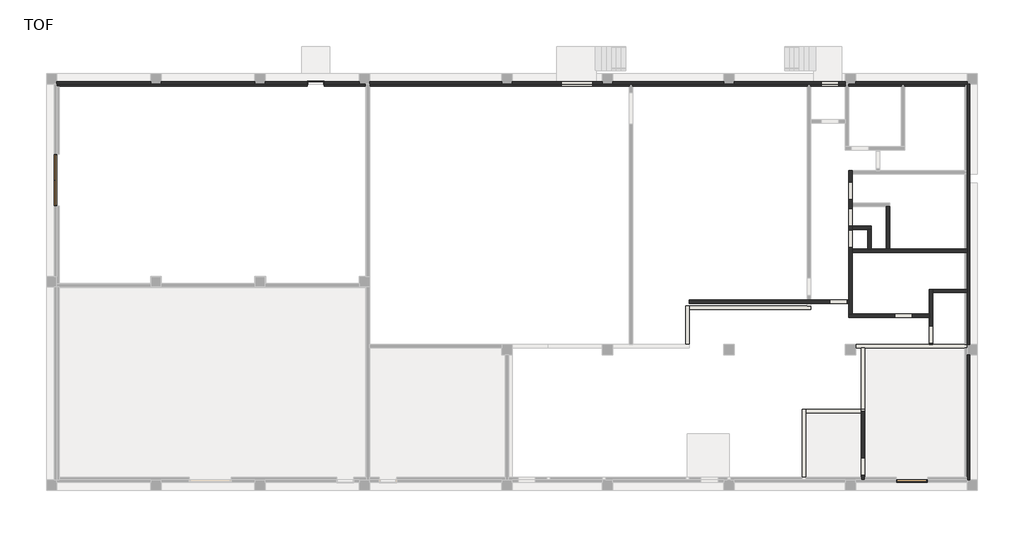
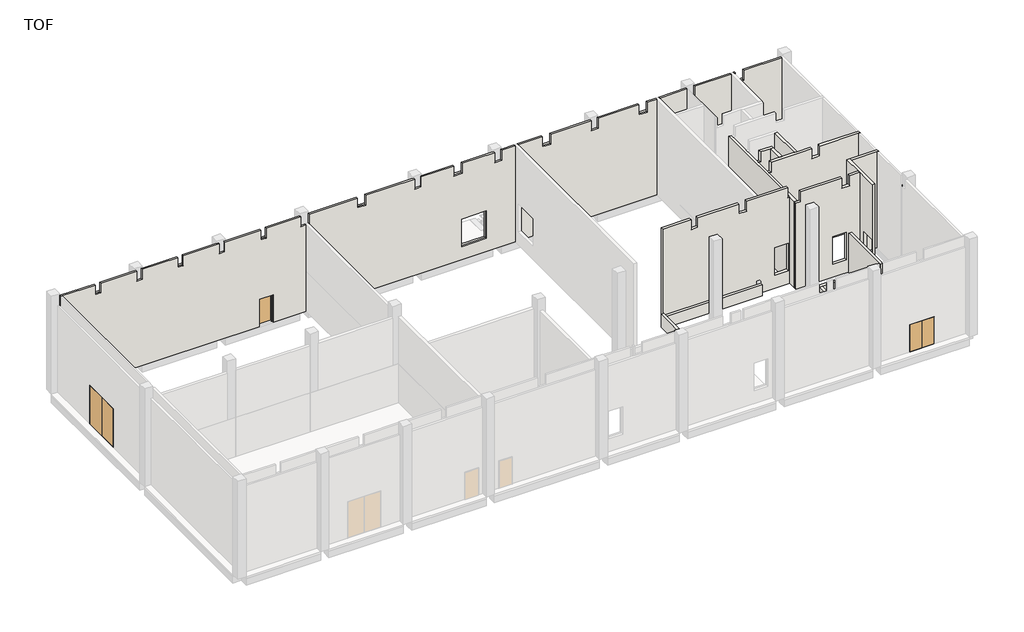
# One storey, part 2 of 4: 19 walls, 3 doors.
"""IFC4 building model written with IfcOpenShell, lengths in millimetres."""

import ifcopenshell
import ifcopenshell.guid

model = None  # the IFC model being written
_history = None  # IfcOwnerHistory: only IFC2X3 demands one
_inside = {}  # id of a spatial element -> (the spatial element, [elements in it])
_under = {}  # id of a project, library or spatial element -> (it, [spatial elements below it])
_declared = {}  # id of a project -> (the project, [libraries it declares])
_typed = {}  # id of a type object -> (the type object, [elements of that type])
_made_of = {}  # id of a material, layer set ... -> (it, [elements and type objects made of it])


def new_model(schema):
    """Start an empty IFC model of exactly this schema.

    Asked for "IFC4X3", IfcOpenShell would pick the latest addendum, in which some entities
    have other attributes; the version numbers below select the first issue.
    IFC2X3 requires an IfcOwnerHistory on every rooted entity: one is made here for all.
    """
    global model, _history
    if schema == "IFC4X3":
        model = ifcopenshell.file(schema_version=(4, 3, 0, 0))
    else:
        model = ifcopenshell.file(schema=schema)
    _inside.clear()
    _under.clear()
    _declared.clear()
    _typed.clear()
    _made_of.clear()
    _history = None
    if model.schema == "IFC2X3":
        org = make("IfcOrganization", Name="unknown")
        user = make(
            "IfcPersonAndOrganization",
            ThePerson=make("IfcPerson", FamilyName="unknown"),
            TheOrganization=org,
        )
        app = make(
            "IfcApplication",
            ApplicationDeveloper=org,
            Version="unknown",
            ApplicationFullName="unknown",
            ApplicationIdentifier="unknown",
        )
        _history = make(
            "IfcOwnerHistory",
            OwningUser=user,
            OwningApplication=app,
            ChangeAction="ADDED",
            CreationDate=0,
        )
    return model


def make(cls, **values):
    """One entity of the class cls with the attributes given. An attribute that is None is left unset."""
    return model.create_entity(
        cls, **{name: value for name, value in values.items() if value is not None}
    )


def rooted(cls, **values):
    """An entity with a GlobalId (a new one), such as an element, a storey or a relation."""
    return make(cls, GlobalId=ifcopenshell.guid.new(), OwnerHistory=_history, **values)


def si_unit(unit_type, name, prefix=None):
    """IfcSIUnit, for example si_unit("LENGTHUNIT", "METRE", prefix="MILLI")."""
    return make("IfcSIUnit", UnitType=unit_type, Prefix=prefix, Name=name)


def assignment(units):
    """IfcUnitAssignment: the units of a project."""
    return None if units is None else make("IfcUnitAssignment", Units=units)


def point(xyz):
    """IfcCartesianPoint."""
    return None if xyz is None else make("IfcCartesianPoint", Coordinates=xyz)


def direction(xyz):
    """IfcDirection."""
    return None if xyz is None else make("IfcDirection", DirectionRatios=xyz)


def frame(location, z_axis=None, x_axis=None):
    """IfcAxis2Placement3D, a coordinate frame: its origin and axes. An axis left out is left unset."""
    return make(
        "IfcAxis2Placement3D",
        Location=point(location),
        Axis=direction(z_axis),
        RefDirection=direction(x_axis),
    )


def origin():
    """The frame at (0, 0, 0) with its axes left unset."""
    return frame((0.0, 0.0, 0.0))


def origin_with_axes():
    """The frame at (0, 0, 0) with the z axis (0, 0, 1) and the x axis (1, 0, 0) written out."""
    return frame((0.0, 0.0, 0.0), z_axis=(0.0, 0.0, 1.0), x_axis=(1.0, 0.0, 0.0))


def place(relative_to, where):
    """IfcLocalPlacement: puts the frame where relative to a parent placement (None: the world)."""
    return make(
        "IfcLocalPlacement", PlacementRelTo=relative_to, RelativePlacement=where
    )


def context(
    kind, dimensions, precision=None, world=None, true_north=None, identifier=None
):
    """IfcGeometricRepresentationContext, for example the 3D "Model" context."""
    return make(
        "IfcGeometricRepresentationContext",
        ContextIdentifier=identifier,
        ContextType=kind,
        CoordinateSpaceDimension=dimensions,
        Precision=precision,
        WorldCoordinateSystem=world,
        TrueNorth=true_north,
    )


def project(units=None, contexts=None):
    """IfcProject with its units and contexts."""
    return rooted(
        "IfcProject",
        Name="project",
        RepresentationContexts=contexts,
        UnitsInContext=assignment(units),
    )


def spatial(cls, under=None, at=None, **own):
    """A site, building, storey or space (cls), placed at a placement, below another one or the project."""
    s = rooted(cls, ObjectPlacement=at, **own)
    if under is not None:
        _under.setdefault(under.id(), (under, []))[1].append(s)
    return s


def polyline(points):
    """IfcPolyline through the points."""
    return make("IfcPolyline", Points=[point(p) for p in points])


def outline(outer, holes=None, kind="AREA"):
    """IfcArbitraryClosedProfileDef: a profile drawn as a closed curve; with holes, ...WithVoids."""
    if holes is None:
        return make("IfcArbitraryClosedProfileDef", ProfileType=kind, OuterCurve=outer)
    return make(
        "IfcArbitraryProfileDefWithVoids",
        ProfileType=kind,
        OuterCurve=outer,
        InnerCurves=holes,
    )


def extrude(swept, where, along, depth):
    """IfcExtrudedAreaSolid: the profile swept, set in the frame where, extruded along a direction by depth."""
    return make(
        "IfcExtrudedAreaSolid",
        SweptArea=swept,
        Position=where,
        ExtrudedDirection=direction(along),
        Depth=depth,
    )


def faces_of(points, faces, orient=None, outer=None):
    """IfcFace entities. A face is a list of loops; a loop is a list of indices into points, from 0.

    orient and outer hold one flag for each loop. By default every Orientation is true, the
    first loop of a face is its IfcFaceOuterBound and the others are IfcFaceBound.
    """
    made = []
    for i, loops in enumerate(faces):
        bounds = []
        for j, loop in enumerate(loops):
            is_outer = j == 0 if outer is None else outer[i][j]
            bounds.append(
                make(
                    "IfcFaceOuterBound" if is_outer else "IfcFaceBound",
                    Bound=make("IfcPolyLoop", Polygon=[points[k] for k in loop]),
                    Orientation=True if orient is None else orient[i][j],
                )
            )
        made.append(make("IfcFace", Bounds=bounds))
    return made


def faceted_brep(points, faces, orient=None, outer=None, voids=None):
    """IfcFacetedBrep: a solid bounded by flat faces; with voids (closed shells), ...WithVoids."""
    shared = [point(p) for p in points]
    hull = make("IfcClosedShell", CfsFaces=faces_of(shared, faces, orient, outer))
    if voids is None:
        return make("IfcFacetedBrep", Outer=hull)
    return make(
        "IfcFacetedBrepWithVoids",
        Outer=hull,
        Voids=[
            make(cls, CfsFaces=faces_of(shared, fs, o, b)) for cls, fs, o, b in voids
        ],
    )


def shape(context_of_items, identifier, shape_type, items):
    """IfcShapeRepresentation: the items that make up one representation, for example the "Body"."""
    return make(
        "IfcShapeRepresentation",
        ContextOfItems=context_of_items,
        RepresentationIdentifier=identifier,
        RepresentationType=shape_type,
        Items=items,
    )


def source(mapping_origin, context_of_items, identifier, shape_type, items):
    """IfcRepresentationMap: a shape defined once, which mapped items show again and again."""
    return make(
        "IfcRepresentationMap",
        MappingOrigin=mapping_origin,
        MappedRepresentation=shape(context_of_items, identifier, shape_type, items),
    )


def transform(
    local_origin,
    x_axis=None,
    y_axis=None,
    z_axis=None,
    scale=None,
    scale2=None,
    scale3=None,
    uniform=True,
):
    """IfcCartesianTransformationOperator3D, or its non-uniform kind. x_axis, y_axis, z_axis: its Axis1, 2, 3."""
    if uniform:
        return make(
            "IfcCartesianTransformationOperator3D",
            Axis1=direction(x_axis),
            Axis2=direction(y_axis),
            LocalOrigin=point(local_origin),
            Scale=scale,
            Axis3=direction(z_axis),
        )
    return make(
        "IfcCartesianTransformationOperator3DnonUniform",
        Axis1=direction(x_axis),
        Axis2=direction(y_axis),
        LocalOrigin=point(local_origin),
        Scale=scale,
        Axis3=direction(z_axis),
        Scale2=scale2,
        Scale3=scale3,
    )


def mapped(mapping_source, mapping_target):
    """IfcMappedItem: shows the shape of a source again, moved by a transform."""
    return make(
        "IfcMappedItem", MappingSource=mapping_source, MappingTarget=mapping_target
    )


def made_of(thing, what):
    """Note that an element or type object is made of a material, layer set ...; save() writes the relation."""
    if what is not None:
        _made_of.setdefault(what.id(), (what, []))[1].append(thing)
    return thing


def element(
    cls,
    number,
    at=None,
    inside=None,
    cuts=None,
    type_object=None,
    material=None,
    context=None,
    identifier="Body",
    shape_type=None,
    held_by="IfcProductDefinitionShape",
    body=None,
    shapes=None,
    **own,
):
    """One element of the class cls, such as IfcWall. Its Tag is "e" and its number.

    at: its placement. inside: the storey or other place that contains it. cuts: it is an
    opening in that element (IfcRelVoidsElement). A single representation is given by context,
    identifier, shape_type and body (its items); several are given by shapes. held_by: the class
    of the entity that holds the representations. save() writes the other relations.
    """
    e = rooted(cls, Tag="e%d" % number, ObjectPlacement=at, **own)
    if body is not None:
        shapes = [shape(context, identifier, shape_type, body)]
    if shapes is not None:
        e.Representation = make(held_by, Representations=shapes)
    if inside is not None:
        _inside.setdefault(inside.id(), (inside, []))[1].append(e)
    if cuts is not None:
        rooted(
            "IfcRelVoidsElement", RelatingBuildingElement=cuts, RelatedOpeningElement=e
        )
    if type_object is not None:
        _typed.setdefault(type_object.id(), (type_object, []))[1].append(e)
    return made_of(e, material)


def aggregate(whole, parts):
    """IfcRelAggregates: a whole, such as a stair, and the parts it consists of."""
    return rooted("IfcRelAggregates", RelatingObject=whole, RelatedObjects=parts)


def save(model, path):
    """Write the relations noted so far, then the file.

    IfcRelAggregates (storeys below a building ...), IfcRelContainedInSpatialStructure (elements
    in a storey), IfcRelDefinesByType, IfcRelAssociatesMaterial and IfcRelDeclares: one each for
    every whole, place, type object, material and project.
    """
    for whole, parts in _under.values():
        aggregate(whole, parts)
    for where, things in _inside.values():
        rooted(
            "IfcRelContainedInSpatialStructure",
            RelatedElements=things,
            RelatingStructure=where,
        )
    for kind, things in _typed.values():
        rooted("IfcRelDefinesByType", RelatedObjects=things, RelatingType=kind)
    for what, things in _made_of.values():
        rooted("IfcRelAssociatesMaterial", RelatedObjects=things, RelatingMaterial=what)
    for by, libraries in _declared.values():
        rooted("IfcRelDeclares", RelatingContext=by, RelatedDefinitions=libraries)
    model.write(path)


def double_door_steel_580823b0(model_context):
    return source(origin(), model_context, "Body", "SolidModel", [
        extrude(outline(polyline([(880.0, 35.0), (0.0, 35.0), (0.0, 75.0), (880.0, 75.0), (880.0, 35.0)])), frame((0.0, 0.0, 20.0), z_axis=(0.0, 0.0, 1.0), x_axis=(1.0, 0.0, 0.0)), (0.0, 0.0, 1.0), 2060.0),
        extrude(outline(polyline([(0.0, 35.0), (-880.0, 35.0), (-880.0, 75.0), (0.0, 75.0), (0.0, 35.0)])), frame((0.0, 0.0, 20.0), z_axis=(0.0, 0.0, 1.0), x_axis=(1.0, 0.0, 0.0)), (0.0, 0.0, 1.0), 2060.0),
        faceted_brep([(900.0, -75.0, 2100.0), (900.0, 75.0, 2100.0), (-900.0, 75.0, 2100.0), (-900.0, -75.0, 2100.0), (865.0, 35.0, 2065.0), (865.0, -75.0, 2065.0), (-865.0, -75.0, 2065.0), (-865.0, 35.0, 2065.0), (880.0, 75.0, 2080.0), (880.0, 35.0, 2080.0), (-880.0, 35.0, 2080.0), (-880.0, 75.0, 2080.0), (-900.0, 75.0, 0.0), (-900.0, -75.0, 0.0), (-865.0, -75.0, 35.0), (-865.0, 35.0, 35.0), (-880.0, 35.0, 20.0), (-880.0, 75.0, 20.0), (900.0, 75.0, 0.0), (880.0, 75.0, 20.0), (900.0, -75.0, 0.0), (865.0, -75.0, 35.0), (865.0, 35.0, 35.0), (880.0, 35.0, 20.0)], [[[0, 1, 2, 3]], [[4, 5, 6, 7]], [[8, 9, 10, 11]], [[3, 2, 12, 13]], [[7, 6, 14, 15]], [[11, 10, 16, 17]], [[18, 12, 2, 1], [8, 11, 17, 19]], [[13, 12, 18, 20]], [[0, 3, 13, 20], [21, 14, 6, 5]], [[15, 14, 21, 22]], [[23, 16, 10, 9], [4, 7, 15, 22]], [[17, 16, 23, 19]], [[20, 18, 1, 0]], [[22, 21, 5, 4]], [[19, 23, 9, 8]]]),
    ])


def double_door_steel_0432cfbf(model_context):
    return source(origin(), model_context, "Body", "SolidModel", [
        extrude(outline(polyline([(1480.0, 35.0), (0.0, 35.0), (0.0, 75.0), (1480.0, 75.0), (1480.0, 35.0)])), frame((0.0, 0.0, 20.0), z_axis=(0.0, 0.0, 1.0), x_axis=(1.0, 0.0, 0.0)), (0.0, 0.0, 1.0), 2960.0),
        extrude(outline(polyline([(0.0, 35.0), (-1480.0, 35.0), (-1480.0, 75.0), (0.0, 75.0), (0.0, 35.0)])), frame((0.0, 0.0, 20.0), z_axis=(0.0, 0.0, 1.0), x_axis=(1.0, 0.0, 0.0)), (0.0, 0.0, 1.0), 2960.0),
        faceted_brep([(1500.0, -75.0, 3000.0), (1500.0, 75.0, 3000.0), (-1500.0, 75.0, 3000.0), (-1500.0, -75.0, 3000.0), (1465.0, 35.0, 2965.0), (1465.0, -75.0, 2965.0), (-1465.0, -75.0, 2965.0), (-1465.0, 35.0, 2965.0), (1480.0, 75.0, 2980.0), (1480.0, 35.0, 2980.0), (-1480.0, 35.0, 2980.0), (-1480.0, 75.0, 2980.0), (-1500.0, 75.0, 0.0), (-1500.0, -75.0, 0.0), (-1465.0, -75.0, 35.0), (-1465.0, 35.0, 35.0), (-1480.0, 35.0, 20.0), (-1480.0, 75.0, 20.0), (1500.0, 75.0, 0.0), (1480.0, 75.0, 20.0), (1500.0, -75.0, 0.0), (1465.0, -75.0, 35.0), (1465.0, 35.0, 35.0), (1480.0, 35.0, 20.0)], [[[0, 1, 2, 3]], [[4, 5, 6, 7]], [[8, 9, 10, 11]], [[3, 2, 12, 13]], [[7, 6, 14, 15]], [[11, 10, 16, 17]], [[18, 12, 2, 1], [8, 11, 17, 19]], [[13, 12, 18, 20]], [[0, 3, 13, 20], [21, 14, 6, 5]], [[15, 14, 21, 22]], [[23, 16, 10, 9], [4, 7, 15, 22]], [[17, 16, 23, 19]], [[20, 18, 1, 0]], [[22, 21, 5, 4]], [[19, 23, 9, 8]]]),
    ])


def single_door_steel_8d57826b(model_context):
    return source(origin(), model_context, "Body", "SolidModel", [
        extrude(outline(polyline([(470.0, -105.0), (-470.0, -105.0), (-470.0, -70.0), (470.0, -70.0), (470.0, -105.0)])), origin_with_axes(), (0.0, 0.0, 1.0), 2070.0),
        faceted_brep([(470.0, -105.0, 0.0), (470.0, -70.0, 0.0), (450.0, -70.0, 0.0), (450.0, 70.0, 0.0), (470.0, 70.0, 0.0), (470.0, 105.0, 0.0), (500.0, 105.0, 0.0), (500.0, -105.0, 0.0), (500.0, -105.0, 2100.0), (-500.0, -105.0, 2100.0), (-500.0, -105.0, 0.0), (-470.0, -105.0, 0.0), (-470.0, -105.0, 2070.0), (470.0, -105.0, 2070.0), (500.0, 105.0, 2100.0), (470.0, 105.0, 2070.0), (-470.0, 105.0, 2070.0), (-470.0, 105.0, 0.0), (-500.0, 105.0, 0.0), (-500.0, 105.0, 2100.0), (470.0, 70.0, 2070.0), (450.0, 70.0, 2050.0), (-450.0, 70.0, 2050.0), (-450.0, 70.0, 0.0), (-470.0, 70.0, 0.0), (-470.0, 70.0, 2070.0), (450.0, -70.0, 2050.0), (470.0, -70.0, 2070.0), (-470.0, -70.0, 2070.0), (-470.0, -70.0, 0.0), (-450.0, -70.0, 0.0), (-450.0, -70.0, 2050.0)], [[[0, 1, 2, 3, 4, 5, 6, 7]], [[7, 8, 9, 10, 11, 12, 13, 0]], [[6, 14, 8, 7]], [[5, 15, 16, 17, 18, 19, 14, 6]], [[4, 20, 15, 5]], [[3, 21, 22, 23, 24, 25, 20, 4]], [[2, 26, 21, 3]], [[1, 27, 28, 29, 30, 31, 26, 2]], [[0, 13, 27, 1]], [[12, 11, 29, 28]], [[11, 10, 18, 17, 24, 23, 30, 29]], [[19, 18, 10, 9]], [[25, 24, 17, 16]], [[31, 30, 23, 22]], [[14, 19, 9, 8]], [[20, 25, 16, 15]], [[26, 31, 22, 21]], [[13, 12, 28, 27]]]),
    ])


model = new_model("IFC4")

# Units and contexts
model_context = context("Model", 3, world=origin())
ifc_project = project(units=[si_unit("LENGTHUNIT", "METRE", prefix="MILLI")], contexts=[model_context])

# Site, building, storey
site = spatial("IfcSite", under=ifc_project)
building = spatial("IfcBuilding", under=site)
storey = spatial("IfcBuildingStorey", under=building, Name="TOF", Elevation=149.9618634)

# Doors
placement = place(None, origin())
double_door_steel_shape = double_door_steel_580823b0(model_context)
element("IfcDoor", 1, ObjectType="Double Door_Steel : H_DR_AR_B12_Double Door_Steel_W2000xH2100", at=placement, inside=storey, context=model_context, shape_type="MappedRepresentation", body=[
    mapped(double_door_steel_shape, transform((49525.0, 724.5208589, 149.9618634), x_axis=(-1.0, 0.0, 0.0), y_axis=(0.0, -1.0, 0.0), z_axis=(0.0, 0.0, 1.0))),
])
double_door_steel_2_shape = double_door_steel_0432cfbf(model_context)
element("IfcDoor", 2, ObjectType="Double Door_Steel : H_DR_AR_B12_Double Door_Steel_W3000xH3000", at=placement, inside=storey, context=model_context, shape_type="MappedRepresentation", body=[
    mapped(double_door_steel_2_shape, transform((225.0, 18074.5208589, 149.9618634), x_axis=(0.0, 1.0, 0.0), y_axis=(-1.0, 0.0, 0.0), z_axis=(0.0, 0.0, 1.0))),
])
single_door_steel_shape = single_door_steel_8d57826b(model_context)
element("IfcDoor", 3, ObjectType="Single Door_Steel : H_DR_AR_B12_Single Door_Steel_W1000xH2100", at=placement, inside=storey, context=model_context, shape_type="MappedRepresentation", body=[
    mapped(single_door_steel_shape, transform((15200.0, 23674.5208589, 149.9618634), x_axis=(-1.0, 0.0, 0.0), y_axis=(0.0, -1.0, 0.0), z_axis=(0.0, 0.0, 1.0))),
])

# Walls
element("IfcWall", 4, ObjectType="H_WA_AR_B02_Ext Wall_RC T150", at=placement, inside=storey, context=model_context, shape_type="Brep", body=[
    faceted_brep([(14700.0, 23599.5208589, 149.9618634), (14700.0, 23599.5208589, 2249.9618634), (15700.0, 23599.5208589, 2249.9618634), (15700.0, 23599.5208589, 149.9618634), (17700.0, 23599.5208589, 149.9618634), (17700.0, 23599.5208589, 6749.9618634), (15200.0, 23599.5208589, 6749.9618634), (14800.0, 23599.5208589, 6749.9618634), (12300.0, 23599.5208589, 6749.9618634), (12300.0, 23599.5208589, 149.9618634), (14700.0, 23749.5208589, 2249.9618634), (14700.0, 23749.5208589, 149.9618634), (12300.0, 23749.5208589, 149.9618634), (12300.0, 23749.5208589, 6749.9618634), (17700.0, 23749.5208589, 6749.9618634), (17700.0, 23749.5208589, 149.9618634), (15700.0, 23749.5208589, 149.9618634), (15700.0, 23749.5208589, 2249.9618634)], [[[0, 1, 2, 3, 4, 5, 6, 7, 8, 9]], [[10, 11, 12, 13, 14, 15, 16, 17]], [[11, 0, 9, 12]], [[3, 16, 15, 4]], [[10, 1, 0, 11]], [[1, 10, 17, 2]], [[2, 17, 16, 3]], [[12, 9, 8, 13]], [[4, 15, 14, 5]], [[8, 7, 6, 5, 14, 13]]]),
    faceted_brep([(300.0, 23599.5208589, 149.9618634), (5700.0, 23599.5208589, 149.9618634), (5700.0, 23599.5208589, 6749.9618634), (3200.0, 23599.5208589, 6749.9618634), (2800.0, 23599.5208589, 6749.9618634), (300.0, 23599.5208589, 6749.9618634), (5700.0, 23749.5208589, 149.9618634), (300.0, 23749.5208589, 149.9618634), (300.0, 23749.5208589, 6749.9618634), (5700.0, 23749.5208589, 6749.9618634)], [[[0, 1, 2, 3, 4, 5]], [[6, 7, 8, 9]], [[0, 7, 6, 1]], [[7, 0, 5, 8]], [[1, 6, 9, 2]], [[5, 4, 3, 2, 9, 8]]]),
    faceted_brep([(6300.0, 23599.5208589, 149.9618634), (11700.0, 23599.5208589, 149.9618634), (11700.0, 23599.5208589, 6749.9618634), (9200.0, 23599.5208589, 6749.9618634), (8800.0, 23599.5208589, 6749.9618634), (6300.0, 23599.5208589, 6749.9618634), (11700.0, 23749.5208589, 149.9618634), (6300.0, 23749.5208589, 149.9618634), (6300.0, 23749.5208589, 6749.9618634), (11700.0, 23749.5208589, 6749.9618634)], [[[0, 1, 2, 3, 4, 5]], [[6, 7, 8, 9]], [[0, 7, 6, 1]], [[7, 0, 5, 8]], [[1, 6, 9, 2]], [[5, 4, 3, 2, 9, 8]]]),
    faceted_brep([(18300.0, 23599.5208589, 149.9618634), (25900.0, 23599.5208589, 149.9618634), (25900.0, 23599.5208589, 6749.9618634), (22400.0, 23599.5208589, 6749.9618634), (21800.0, 23599.5208589, 6749.9618634), (18300.0, 23599.5208589, 6749.9618634), (25900.0, 23749.5208589, 149.9618634), (18300.0, 23749.5208589, 149.9618634), (18300.0, 23749.5208589, 6749.9618634), (25900.0, 23749.5208589, 6749.9618634)], [[[0, 1, 2, 3, 4, 5]], [[6, 7, 8, 9]], [[0, 7, 6, 1]], [[7, 0, 5, 8]], [[1, 6, 9, 2]], [[5, 4, 3, 2, 9, 8]]]),
    faceted_brep([(26500.0, 23599.5208589, 149.9618634), (31700.0, 23599.5208589, 149.9618634), (31700.0, 23599.5208589, 6749.9618634), (29400.0, 23599.5208589, 6749.9618634), (28800.0, 23599.5208589, 6749.9618634), (26500.0, 23599.5208589, 6749.9618634), (31150.0, 23599.5208589, 3249.9618634), (31150.0, 23599.5208589, 1149.9618634), (29350.0, 23599.5208589, 1149.9618634), (29350.0, 23599.5208589, 3249.9618634), (31700.0, 23749.5208589, 149.9618634), (26500.0, 23749.5208589, 149.9618634), (26500.0, 23749.5208589, 6749.9618634), (31700.0, 23749.5208589, 6749.9618634), (31150.0, 23749.5208589, 1149.9618634), (31150.0, 23749.5208589, 3249.9618634), (29350.0, 23749.5208589, 3249.9618634), (29350.0, 23749.5208589, 1149.9618634)], [[[0, 1, 2, 3, 4, 5], [6, 7, 8, 9]], [[10, 11, 12, 13], [14, 15, 16, 17]], [[0, 11, 10, 1]], [[15, 14, 7, 6]], [[16, 15, 6, 9]], [[17, 16, 9, 8]], [[14, 17, 8, 7]], [[11, 0, 5, 12]], [[1, 10, 13, 2]], [[5, 4, 3, 2, 13, 12]]]),
    faceted_brep([(32300.0, 23599.5208589, 149.9618634), (33250.0, 23599.5208589, 149.9618634), (33450.0, 23599.5208589, 149.9618634), (38700.0, 23599.5208589, 149.9618634), (38700.0, 23599.5208589, 6749.9618634), (35800.0, 23599.5208589, 6749.9618634), (35200.0, 23599.5208589, 6749.9618634), (32300.0, 23599.5208589, 6749.9618634), (38700.0, 23749.5208589, 149.9618634), (32300.0, 23749.5208589, 149.9618634), (32300.0, 23749.5208589, 6749.9618634), (38700.0, 23749.5208589, 6749.9618634)], [[[0, 1, 2, 3, 4, 5, 6, 7]], [[8, 9, 10, 11]], [[0, 9, 8, 3, 2, 1]], [[9, 0, 7, 10]], [[3, 8, 11, 4]], [[7, 6, 5, 4, 11, 10]]]),
    faceted_brep([(39300.0, 23599.5208589, 149.9618634), (43500.0, 23599.5208589, 149.9618634), (43700.0, 23599.5208589, 149.9618634), (45700.0, 23599.5208589, 149.9618634), (45700.0, 23599.5208589, 6749.9618634), (42800.0, 23599.5208589, 6749.9618634), (42200.0, 23599.5208589, 6749.9618634), (39300.0, 23599.5208589, 6749.9618634), (44300.0, 23599.5208589, 1149.9618634), (44300.0, 23599.5208589, 3249.9618634), (45300.0, 23599.5208589, 3249.9618634), (45300.0, 23599.5208589, 1149.9618634), (45700.0, 23749.5208589, 149.9618634), (39300.0, 23749.5208589, 149.9618634), (39300.0, 23749.5208589, 6749.9618634), (45700.0, 23749.5208589, 6749.9618634), (44300.0, 23749.5208589, 3249.9618634), (44300.0, 23749.5208589, 1149.9618634), (45300.0, 23749.5208589, 1149.9618634), (45300.0, 23749.5208589, 3249.9618634)], [[[0, 1, 2, 3, 4, 5, 6, 7], [8, 9, 10, 11]], [[12, 13, 14, 15], [16, 17, 18, 19]], [[0, 13, 12, 3, 2, 1]], [[9, 8, 17, 16]], [[10, 9, 16, 19]], [[11, 10, 19, 18]], [[8, 11, 18, 17]], [[13, 0, 7, 14]], [[3, 12, 15, 4]], [[7, 6, 5, 4, 15, 14]]]),
    faceted_brep([(46300.0, 23599.5208589, 149.9618634), (48900.0, 23599.5208589, 149.9618634), (49100.0, 23599.5208589, 149.9618634), (52574.0, 23599.5208589, 149.9618634), (52700.0, 23599.5208589, 149.9618634), (52700.0, 23599.5208589, 6749.9618634), (49800.0, 23599.5208589, 6749.9618634), (49200.0, 23599.5208589, 6749.9618634), (46300.0, 23599.5208589, 6749.9618634), (52700.0, 23749.5208589, 149.9618634), (46300.0, 23749.5208589, 149.9618634), (46300.0, 23749.5208589, 6749.9618634), (52700.0, 23749.5208589, 6749.9618634)], [[[0, 1, 2, 3, 4, 5, 6, 7, 8]], [[9, 10, 11, 12]], [[9, 4, 3, 2, 1, 0, 10]], [[4, 9, 12, 5]], [[10, 0, 8, 11]], [[8, 7, 6, 5, 12, 11]]]),
])
element("IfcWall", 5, ObjectType="H_WA_AR_B02_Ext Wall_RC T150", at=placement, inside=storey, context=model_context, shape_type="Brep", body=[
    faceted_brep([(52700.0, 7999.5208589, 149.9618634), (52700.0, 925.5208589, 149.9618634), (52700.0, 799.5208589, 149.9618634), (52700.0, 799.5208589, 6749.9618634), (52700.0, 7999.5208589, 6749.9618634), (52850.0, 799.5208589, 149.9618634), (52850.0, 7999.5208589, 149.9618634), (52850.0, 7999.5208589, 6749.9618634), (52850.0, 799.5208589, 6749.9618634)], [[[0, 1, 2, 3, 4]], [[5, 6, 7, 8]], [[5, 2, 1, 0, 6]], [[2, 5, 8, 3]], [[6, 0, 4, 7]], [[4, 3, 8, 7]]]),
    faceted_brep([(52700.0, 23599.5208589, 149.9618634), (52700.0, 18599.5208589, 149.9618634), (52700.0, 18399.5208589, 149.9618634), (52700.0, 17899.5208589, 149.9618634), (52700.0, 14099.5208589, 149.9618634), (52700.0, 13899.5208589, 149.9618634), (52700.0, 11774.5208589, 149.9618634), (52700.0, 11574.5208589, 149.9618634), (52700.0, 8599.5208589, 149.9618634), (52700.0, 8599.5208589, 6749.9618634), (52700.0, 23599.5208589, 6749.9618634), (52850.0, 8599.5208589, 149.9618634), (52850.0, 23599.5208589, 149.9618634), (52850.0, 23599.5208589, 6749.9618634), (52850.0, 8599.5208589, 6749.9618634)], [[[0, 1, 2, 3, 4, 5, 6, 7, 8, 9, 10]], [[11, 12, 13, 14]], [[0, 12, 11, 8, 7, 6, 5, 4, 3, 2, 1]], [[12, 0, 10, 13]], [[8, 11, 14, 9]], [[10, 9, 14, 13]]]),
])
element("IfcWall", 6, ObjectType="H_WA_AR_B02_Int Wall_Block T200", at=placement, inside=storey, context=model_context, shape_type="Brep", body=[
    faceted_brep([(36700.0, 10949.5208589, 149.9618634), (45895.0, 10949.5208589, 149.9618634), (45895.0, 10949.5208589, 6749.9618634), (45750.0, 10949.5208589, 6749.9618634), (45750.0, 10949.5208589, 7499.9618634), (42800.0, 10949.5208589, 7499.9618634), (42800.0, 10949.5208589, 6749.9618634), (42200.0, 10949.5208589, 6749.9618634), (42200.0, 10949.5208589, 7499.9618634), (39250.0, 10949.5208589, 7499.9618634), (39250.0, 10949.5208589, 6749.9618634), (38750.0, 10949.5208589, 6749.9618634), (38750.0, 10949.5208589, 7499.9618634), (36700.0, 10949.5208589, 7499.9618634), (44800.0, 10949.5208589, 1149.9618634), (44800.0, 10949.5208589, 3249.9618634), (45800.0, 10949.5208589, 3249.9618634), (45800.0, 10949.5208589, 1149.9618634), (45895.0, 11149.5208589, 149.9618634), (43700.0, 11149.5208589, 149.9618634), (43500.0, 11149.5208589, 149.9618634), (36700.0, 11149.5208589, 149.9618634), (36700.0, 11149.5208589, 1149.9618634), (36700.0, 11149.5208589, 7499.9618634), (38750.0, 11149.5208589, 7499.9618634), (38750.0, 11149.5208589, 6749.9618634), (39250.0, 11149.5208589, 6749.9618634), (39250.0, 11149.5208589, 7499.9618634), (42200.0, 11149.5208589, 7499.9618634), (42200.0, 11149.5208589, 6749.9618634), (42800.0, 11149.5208589, 6749.9618634), (42800.0, 11149.5208589, 7499.9618634), (43500.0, 11149.5208589, 7499.9618634), (43700.0, 11149.5208589, 7499.9618634), (45750.0, 11149.5208589, 7499.9618634), (45750.0, 11149.5208589, 6749.9618634), (45895.0, 11149.5208589, 6749.9618634), (44800.0, 11149.5208589, 3249.9618634), (44800.0, 11149.5208589, 1149.9618634), (45800.0, 11149.5208589, 1149.9618634), (45800.0, 11149.5208589, 3249.9618634)], [[[0, 1, 2, 3, 4, 5, 6, 7, 8, 9, 10, 11, 12, 13], [14, 15, 16, 17]], [[18, 19, 20, 21, 22, 23, 24, 25, 26, 27, 28, 29, 30, 31, 32, 33, 34, 35, 36], [37, 38, 39, 40]], [[1, 0, 21, 20, 19, 18]], [[21, 0, 13, 23, 22]], [[1, 18, 36, 2]], [[15, 14, 38, 37]], [[16, 15, 37, 40]], [[17, 16, 40, 39]], [[14, 17, 39, 38]], [[26, 10, 9, 27]], [[10, 26, 25, 11]], [[11, 25, 24, 12]], [[35, 3, 2, 36]], [[3, 35, 34, 4]], [[7, 29, 28, 8]], [[29, 7, 6, 30]], [[30, 6, 5, 31]], [[5, 4, 34, 33, 32, 31]], [[9, 8, 28, 27]], [[13, 12, 24, 23]]]),
])
element("IfcWall", 7, ObjectType="H_WA_AR_B02_Int Wall_Block T200", at=placement, inside=storey, context=model_context, shape_type="Brep", body=[
    faceted_brep([(46800.0, 799.5208589, 149.9618634), (46800.0, 925.5208589, 149.9618634), (46800.0, 4849.5208589, 149.9618634), (46800.0, 4849.5208589, 1149.9618634), (46800.0, 4749.5208589, 1149.9618634), (46800.0, 4749.5208589, 7499.9618634), (46800.0, 925.5208589, 7499.9618634), (46800.0, 799.5208589, 7499.9618634), (46800.0, 2049.5208589, 3249.9618634), (46800.0, 2049.5208589, 1149.9618634), (46800.0, 1049.5208589, 1149.9618634), (46800.0, 1049.5208589, 3249.9618634), (46600.0, 4849.5208589, 149.9618634), (46600.0, 4649.5208589, 149.9618634), (46600.0, 925.5208589, 149.9618634), (46600.0, 799.5208589, 149.9618634), (46600.0, 799.5208589, 7499.9618634), (46600.0, 925.5208589, 7499.9618634), (46600.0, 4649.5208589, 7499.9618634), (46600.0, 4749.5208589, 7499.9618634), (46600.0, 4749.5208589, 1149.9618634), (46600.0, 4849.5208589, 1149.9618634), (46600.0, 2049.5208589, 1149.9618634), (46600.0, 2049.5208589, 3249.9618634), (46600.0, 1049.5208589, 3249.9618634), (46600.0, 1049.5208589, 1149.9618634)], [[[0, 1, 2, 3, 4, 5, 6, 7], [8, 9, 10, 11]], [[12, 13, 14, 15, 16, 17, 18, 19, 20, 21], [22, 23, 24, 25]], [[2, 1, 0, 15, 14, 13, 12]], [[15, 0, 7, 16]], [[23, 22, 9, 8]], [[24, 23, 8, 11]], [[25, 24, 11, 10]], [[22, 25, 10, 9]], [[7, 6, 5, 19, 18, 17, 16]], [[4, 20, 19, 5]], [[20, 4, 3, 21]], [[3, 2, 12, 21]]]),
])
element("IfcWall", 8, ObjectType="H_WA_AR_B02_Int Wall_Block T200", at=placement, inside=storey, context=model_context, shape_type="Brep", body=[
    faceted_brep([(45895.0, 10149.5208589, 149.9618634), (50525.0, 10149.5208589, 149.9618634), (50525.0, 10149.5208589, 7499.9618634), (49800.0, 10149.5208589, 7499.9618634), (49800.0, 10149.5208589, 6749.9618634), (49200.0, 10149.5208589, 6749.9618634), (49200.0, 10149.5208589, 7499.9618634), (46250.0, 10149.5208589, 7499.9618634), (46250.0, 10149.5208589, 6749.9618634), (45895.0, 10149.5208589, 6749.9618634), (49550.0, 10149.5208589, 3249.9618634), (49550.0, 10149.5208589, 1149.9618634), (48550.0, 10149.5208589, 1149.9618634), (48550.0, 10149.5208589, 3249.9618634), (50525.0, 10349.5208589, 149.9618634), (46095.0, 10349.5208589, 149.9618634), (45895.0, 10349.5208589, 149.9618634), (45895.0, 10349.5208589, 6749.9618634), (46095.0, 10349.5208589, 6749.9618634), (46250.0, 10349.5208589, 6749.9618634), (46250.0, 10349.5208589, 7499.9618634), (49200.0, 10349.5208589, 7499.9618634), (49200.0, 10349.5208589, 6749.9618634), (49800.0, 10349.5208589, 6749.9618634), (49800.0, 10349.5208589, 7499.9618634), (50525.0, 10349.5208589, 7499.9618634), (49550.0, 10349.5208589, 1149.9618634), (49550.0, 10349.5208589, 3249.9618634), (48550.0, 10349.5208589, 3249.9618634), (48550.0, 10349.5208589, 1149.9618634)], [[[0, 1, 2, 3, 4, 5, 6, 7, 8, 9], [10, 11, 12, 13]], [[14, 15, 16, 17, 18, 19, 20, 21, 22, 23, 24, 25], [26, 27, 28, 29]], [[1, 0, 16, 15, 14]], [[16, 0, 9, 17]], [[1, 14, 25, 2]], [[27, 26, 11, 10]], [[28, 27, 10, 13]], [[29, 28, 13, 12]], [[26, 29, 12, 11]], [[19, 8, 7, 20]], [[8, 19, 18, 17, 9]], [[5, 22, 21, 6]], [[22, 5, 4, 23]], [[23, 4, 3, 24]], [[3, 2, 25, 24]], [[7, 6, 21, 20]]]),
])
element("IfcWall", 9, ObjectType="H_WA_AR_B02_Int Wall_Block T200", at=placement, inside=storey, context=model_context, shape_type="Brep", body=[
    faceted_brep([(46095.0, 10349.5208589, 149.9618634), (46095.0, 13899.5208589, 149.9618634), (46095.0, 14099.5208589, 149.9618634), (46095.0, 15214.5208589, 149.9618634), (46095.0, 15414.5208589, 149.9618634), (46095.0, 16549.5208589, 149.9618634), (46095.0, 16749.5208589, 149.9618634), (46095.0, 18399.5208589, 149.9618634), (46095.0, 18599.5208589, 149.9618634), (46095.0, 18599.5208589, 6749.9618634), (46095.0, 18399.5208589, 6749.9618634), (46095.0, 16749.5208589, 6749.9618634), (46095.0, 16549.5208589, 6749.9618634), (46095.0, 15414.5208589, 6749.9618634), (46095.0, 15214.5208589, 6749.9618634), (46095.0, 14099.5208589, 6749.9618634), (46095.0, 13899.5208589, 6749.9618634), (46095.0, 10349.5208589, 6749.9618634), (46095.0, 16949.5208589, 1149.9618634), (46095.0, 16949.5208589, 3249.9618634), (46095.0, 17949.5208589, 3249.9618634), (46095.0, 17949.5208589, 1149.9618634), (46095.0, 15412.0208589, 1149.9618634), (46095.0, 15412.0208589, 3249.9618634), (46095.0, 16412.0208589, 3249.9618634), (46095.0, 16412.0208589, 1149.9618634), (46095.0, 15174.5208589, 3249.9618634), (46095.0, 15174.5208589, 1149.9618634), (46095.0, 14174.5208589, 1149.9618634), (46095.0, 14174.5208589, 3249.9618634), (45895.0, 18599.5208589, 149.9618634), (45895.0, 11149.5208589, 149.9618634), (45895.0, 10949.5208589, 149.9618634), (45895.0, 10349.5208589, 149.9618634), (45895.0, 10349.5208589, 6749.9618634), (45895.0, 10949.5208589, 6749.9618634), (45895.0, 11149.5208589, 6749.9618634), (45895.0, 18599.5208589, 6749.9618634), (45895.0, 16949.5208589, 3249.9618634), (45895.0, 16949.5208589, 1149.9618634), (45895.0, 17949.5208589, 1149.9618634), (45895.0, 17949.5208589, 3249.9618634), (45895.0, 15412.0208589, 3249.9618634), (45895.0, 15412.0208589, 1149.9618634), (45895.0, 16412.0208589, 1149.9618634), (45895.0, 16412.0208589, 3249.9618634), (45895.0, 15174.5208589, 1149.9618634), (45895.0, 15174.5208589, 3249.9618634), (45895.0, 14174.5208589, 3249.9618634), (45895.0, 14174.5208589, 1149.9618634)], [[[0, 1, 2, 3, 4, 5, 6, 7, 8, 9, 10, 11, 12, 13, 14, 15, 16, 17], [18, 19, 20, 21], [22, 23, 24, 25], [26, 27, 28, 29]], [[30, 31, 32, 33, 34, 35, 36, 37], [38, 39, 40, 41], [42, 43, 44, 45], [46, 47, 48, 49]], [[8, 7, 6, 5, 4, 3, 2, 1, 0, 33, 32, 31, 30]], [[33, 0, 17, 34]], [[8, 30, 37, 9]], [[19, 18, 39, 38]], [[20, 19, 38, 41]], [[21, 20, 41, 40]], [[18, 21, 40, 39]], [[23, 22, 43, 42]], [[24, 23, 42, 45]], [[25, 24, 45, 44]], [[22, 25, 44, 43]], [[47, 46, 27, 26]], [[48, 47, 26, 29]], [[49, 48, 29, 28]], [[46, 49, 28, 27]], [[17, 16, 15, 14, 13, 12, 11, 10, 9, 37, 36, 35, 34]]]),
])
element("IfcWall", 10, ObjectType="H_WA_AR_B02_Int Wall_Block T200", at=placement, inside=storey, context=model_context, shape_type="Brep", body=[
    faceted_brep([(50725.0, 8599.5208589, 149.9618634), (50725.0, 11574.5208589, 149.9618634), (50725.0, 11774.5208589, 149.9618634), (50725.0, 11774.5208589, 7499.9618634), (50725.0, 11574.5208589, 7499.9618634), (50725.0, 8599.5208589, 7499.9618634), (50725.0, 9649.5208589, 3249.9618634), (50725.0, 9649.5208589, 1149.9618634), (50725.0, 8649.5208589, 1149.9618634), (50725.0, 8649.5208589, 3249.9618634), (50525.0, 11774.5208589, 149.9618634), (50525.0, 10349.5208589, 149.9618634), (50525.0, 10149.5208589, 149.9618634), (50525.0, 8599.5208589, 149.9618634), (50525.0, 8599.5208589, 7499.9618634), (50525.0, 10149.5208589, 7499.9618634), (50525.0, 10349.5208589, 7499.9618634), (50525.0, 11774.5208589, 7499.9618634), (50525.0, 9649.5208589, 1149.9618634), (50525.0, 9649.5208589, 3249.9618634), (50525.0, 8649.5208589, 3249.9618634), (50525.0, 8649.5208589, 1149.9618634)], [[[0, 1, 2, 3, 4, 5], [6, 7, 8, 9]], [[10, 11, 12, 13, 14, 15, 16, 17], [18, 19, 20, 21]], [[2, 1, 0, 13, 12, 11, 10]], [[2, 10, 17, 3]], [[18, 7, 6, 19]], [[19, 6, 9, 20]], [[7, 18, 21, 8]], [[8, 21, 20, 9]], [[5, 4, 3, 17, 16, 15, 14]], [[13, 0, 5, 14]]]),
])
element("IfcWall", 11, ObjectType="H_WA_AR_B02_Int Wall_Block T200", at=placement, inside=storey, context=model_context, shape_type="Brep", body=[
    faceted_brep([(50725.0, 11574.5208589, 149.9618634), (52574.0, 11574.5208589, 149.9618634), (52700.0, 11574.5208589, 149.9618634), (52700.0, 11574.5208589, 7499.9618634), (52574.0, 11574.5208589, 7499.9618634), (50725.0, 11574.5208589, 7499.9618634), (52700.0, 11774.5208589, 149.9618634), (52574.0, 11774.5208589, 149.9618634), (50725.0, 11774.5208589, 149.9618634), (50725.0, 11774.5208589, 7499.9618634), (52574.0, 11774.5208589, 7499.9618634), (52700.0, 11774.5208589, 7499.9618634)], [[[0, 1, 2, 3, 4, 5]], [[6, 7, 8, 9, 10, 11]], [[2, 1, 0, 8, 7, 6]], [[8, 0, 5, 9]], [[2, 6, 11, 3]], [[5, 4, 3, 11, 10, 9]]]),
])
element("IfcWall", 12, ObjectType="H_WA_AR_B02_Int Wall_Block T200", at=placement, inside=storey, context=model_context, shape_type="Brep", body=[
    faceted_brep([(46095.0, 13899.5208589, 149.9618634), (52574.0, 13899.5208589, 149.9618634), (52700.0, 13899.5208589, 149.9618634), (52700.0, 13899.5208589, 7499.9618634), (52574.0, 13899.5208589, 7499.9618634), (49800.0, 13899.5208589, 7499.9618634), (49800.0, 13899.5208589, 6749.9618634), (49200.0, 13899.5208589, 6749.9618634), (49200.0, 13899.5208589, 7499.9618634), (46250.0, 13899.5208589, 7499.9618634), (46250.0, 13899.5208589, 6749.9618634), (46095.0, 13899.5208589, 6749.9618634), (52700.0, 14099.5208589, 149.9618634), (52574.0, 14099.5208589, 149.9618634), (48250.0, 14099.5208589, 149.9618634), (48050.0, 14099.5208589, 149.9618634), (47175.0, 14099.5208589, 149.9618634), (46975.0, 14099.5208589, 149.9618634), (46095.0, 14099.5208589, 149.9618634), (46095.0, 14099.5208589, 6749.9618634), (46250.0, 14099.5208589, 6749.9618634), (46250.0, 14099.5208589, 7499.9618634), (46975.0, 14099.5208589, 7499.9618634), (47175.0, 14099.5208589, 7499.9618634), (48050.0, 14099.5208589, 7499.9618634), (48250.0, 14099.5208589, 7499.9618634), (49200.0, 14099.5208589, 7499.9618634), (49200.0, 14099.5208589, 6749.9618634), (49800.0, 14099.5208589, 6749.9618634), (49800.0, 14099.5208589, 7499.9618634), (52574.0, 14099.5208589, 7499.9618634), (52700.0, 14099.5208589, 7499.9618634)], [[[0, 1, 2, 3, 4, 5, 6, 7, 8, 9, 10, 11]], [[12, 13, 14, 15, 16, 17, 18, 19, 20, 21, 22, 23, 24, 25, 26, 27, 28, 29, 30, 31]], [[2, 1, 0, 18, 17, 16, 15, 14, 13, 12]], [[18, 0, 11, 19]], [[2, 12, 31, 3]], [[20, 10, 9, 21]], [[10, 20, 19, 11]], [[7, 27, 26, 8]], [[27, 7, 6, 28]], [[28, 6, 5, 29]], [[9, 8, 26, 25, 24, 23, 22, 21]], [[5, 4, 3, 31, 30, 29]]]),
])
element("IfcWall", 13, ObjectType="H_WA_AR_B02_Int Wall_Block T200", at=placement, inside=storey, context=model_context, shape_type="SweptSolid", body=[
    extrude(outline(polyline([(48050.0, 14099.5208589), (48050.0, 16549.5208589), (48250.0, 16549.5208589), (48250.0, 14099.5208589), (48050.0, 14099.5208589)])), frame((0.0, 0.0, 149.9618634), z_axis=(0.0, 0.0, 1.0), x_axis=(1.0, 0.0, 0.0)), (0.0, 0.0, 1.0), 7350.0),
])
element("IfcWall", 14, ObjectType="H_WA_AR_B02_Int Wall_Block T200", at=placement, inside=storey, context=model_context, shape_type="Brep", body=[
    faceted_brep([(46095.0, 15214.5208589, 149.9618634), (46975.0, 15214.5208589, 149.9618634), (47175.0, 15214.5208589, 149.9618634), (47175.0, 15214.5208589, 7499.9618634), (46975.0, 15214.5208589, 7499.9618634), (46250.0, 15214.5208589, 7499.9618634), (46250.0, 15214.5208589, 6749.9618634), (46095.0, 15214.5208589, 6749.9618634), (47175.0, 15414.5208589, 149.9618634), (46095.0, 15414.5208589, 149.9618634), (46095.0, 15414.5208589, 6749.9618634), (46250.0, 15414.5208589, 6749.9618634), (46250.0, 15414.5208589, 7499.9618634), (47175.0, 15414.5208589, 7499.9618634)], [[[0, 1, 2, 3, 4, 5, 6, 7]], [[8, 9, 10, 11, 12, 13]], [[2, 1, 0, 9, 8]], [[9, 0, 7, 10]], [[2, 8, 13, 3]], [[11, 6, 5, 12]], [[6, 11, 10, 7]], [[5, 4, 3, 13, 12]]]),
])
element("IfcWall", 15, ObjectType="H_WA_AR_B02_Int Wall_Block T200", at=placement, inside=storey, context=model_context, shape_type="SweptSolid", body=[
    extrude(outline(polyline([(46975.0, 14099.5208589), (46975.0, 15214.5208589), (47175.0, 15214.5208589), (47175.0, 14099.5208589), (46975.0, 14099.5208589)])), frame((0.0, 0.0, 149.9618634), z_axis=(0.0, 0.0, 1.0), x_axis=(1.0, 0.0, 0.0)), (0.0, 0.0, 1.0), 7350.0),
])
element("IfcWall", 16, ObjectType="H_WA_AR_B02_Ext Wall_1L Gypsum_Mineral Wool_T110", at=placement, inside=storey, context=model_context, shape_type="Brep", body=[
    faceted_brep([(18100.0, 23473.5208589, 149.9618634), (18100.0, 23473.5208589, 6749.9618634), (17700.0, 23473.5208589, 6749.9618634), (17700.0, 23473.5208589, 7499.9618634), (15200.0, 23473.5208589, 7499.9618634), (15200.0, 23473.5208589, 6749.9618634), (14800.0, 23473.5208589, 6749.9618634), (14800.0, 23473.5208589, 7499.9618634), (12200.0, 23473.5208589, 7499.9618634), (12200.0, 23473.5208589, 6749.9618634), (11800.0, 23473.5208589, 6749.9618634), (11800.0, 23473.5208589, 7499.9618634), (9200.0, 23473.5208589, 7499.9618634), (9200.0, 23473.5208589, 6749.9618634), (8800.0, 23473.5208589, 6749.9618634), (8800.0, 23473.5208589, 7499.9618634), (6200.0, 23473.5208589, 7499.9618634), (6200.0, 23473.5208589, 6749.9618634), (5800.0, 23473.5208589, 6749.9618634), (5800.0, 23473.5208589, 7499.9618634), (3200.0, 23473.5208589, 7499.9618634), (3200.0, 23473.5208589, 6749.9618634), (2800.0, 23473.5208589, 6749.9618634), (2800.0, 23473.5208589, 7499.9618634), (426.0, 23473.5208589, 7499.9618634), (300.0, 23473.5208589, 7499.9618634), (300.0, 23473.5208589, 149.9618634), (426.0, 23473.5208589, 149.9618634), (14700.0, 23473.5208589, 149.9618634), (14700.0, 23473.5208589, 2249.9618634), (15700.0, 23473.5208589, 2249.9618634), (15700.0, 23473.5208589, 149.9618634), (18100.0, 23599.5208589, 6749.9618634), (18100.0, 23599.5208589, 149.9618634), (17700.0, 23599.5208589, 149.9618634), (15700.0, 23599.5208589, 149.9618634), (15700.0, 23599.5208589, 2249.9618634), (14700.0, 23599.5208589, 2249.9618634), (14700.0, 23599.5208589, 149.9618634), (12300.0, 23599.5208589, 149.9618634), (11700.0, 23599.5208589, 149.9618634), (6300.0, 23599.5208589, 149.9618634), (5700.0, 23599.5208589, 149.9618634), (300.0, 23599.5208589, 149.9618634), (300.0, 23599.5208589, 6749.9618634), (300.0, 23599.5208589, 7499.9618634), (2800.0, 23599.5208589, 7499.9618634), (2800.0, 23599.5208589, 6749.9618634), (3200.0, 23599.5208589, 6749.9618634), (3200.0, 23599.5208589, 7499.9618634), (5700.0, 23599.5208589, 7499.9618634), (5800.0, 23599.5208589, 7499.9618634), (5800.0, 23599.5208589, 6749.9618634), (6200.0, 23599.5208589, 6749.9618634), (6200.0, 23599.5208589, 7499.9618634), (6300.0, 23599.5208589, 7499.9618634), (8800.0, 23599.5208589, 7499.9618634), (8800.0, 23599.5208589, 6749.9618634), (9200.0, 23599.5208589, 6749.9618634), (9200.0, 23599.5208589, 7499.9618634), (11700.0, 23599.5208589, 7499.9618634), (11800.0, 23599.5208589, 7499.9618634), (11800.0, 23599.5208589, 6749.9618634), (12200.0, 23599.5208589, 6749.9618634), (12200.0, 23599.5208589, 7499.9618634), (12300.0, 23599.5208589, 7499.9618634), (14800.0, 23599.5208589, 7499.9618634), (14800.0, 23599.5208589, 6749.9618634), (15200.0, 23599.5208589, 6749.9618634), (15200.0, 23599.5208589, 7499.9618634), (17700.0, 23599.5208589, 7499.9618634), (17700.0, 23599.5208589, 6749.9618634)], [[[0, 1, 2, 3, 4, 5, 6, 7, 8, 9, 10, 11, 12, 13, 14, 15, 16, 17, 18, 19, 20, 21, 22, 23, 24, 25, 26, 27, 28, 29, 30, 31]], [[32, 33, 34, 35, 36, 37, 38, 39, 40, 41, 42, 43, 44, 45, 46, 47, 48, 49, 50, 51, 52, 53, 54, 55, 56, 57, 58, 59, 60, 61, 62, 63, 64, 65, 66, 67, 68, 69, 70, 71]], [[26, 43, 42, 41, 40, 39, 38, 28, 27]], [[33, 0, 31, 35, 34]], [[43, 26, 25, 45, 44]], [[1, 0, 33, 32]], [[37, 29, 28, 38]], [[29, 37, 36, 30]], [[30, 36, 35, 31]], [[53, 17, 16, 54]], [[17, 53, 52, 18]], [[18, 52, 51, 19]], [[63, 9, 8, 64]], [[9, 63, 62, 10]], [[10, 62, 61, 11]], [[71, 2, 1, 32]], [[2, 71, 70, 3]], [[22, 47, 46, 23]], [[47, 22, 21, 48]], [[48, 21, 20, 49]], [[14, 57, 56, 15]], [[57, 14, 13, 58]], [[58, 13, 12, 59]], [[6, 67, 66, 7]], [[67, 6, 5, 68]], [[68, 5, 4, 69]], [[4, 3, 70, 69]], [[8, 7, 66, 65, 64]], [[12, 11, 61, 60, 59]], [[16, 15, 56, 55, 54]], [[20, 19, 51, 50, 49]], [[25, 24, 23, 46, 45]]]),
    faceted_brep([(45900.0, 23473.5208589, 6749.9618634), (45900.0, 23473.5208589, 149.9618634), (48900.0, 23473.5208589, 149.9618634), (48900.0, 23473.5208589, 7499.9618634), (46250.0, 23473.5208589, 7499.9618634), (46250.0, 23473.5208589, 6749.9618634), (45900.0, 23599.5208589, 149.9618634), (45900.0, 23599.5208589, 6749.9618634), (46250.0, 23599.5208589, 6749.9618634), (46250.0, 23599.5208589, 7499.9618634), (46300.0, 23599.5208589, 7499.9618634), (48900.0, 23599.5208589, 7499.9618634), (48900.0, 23599.5208589, 149.9618634), (46300.0, 23599.5208589, 149.9618634)], [[[0, 1, 2, 3, 4, 5]], [[6, 7, 8, 9, 10, 11, 12, 13]], [[1, 6, 13, 12, 2]], [[1, 0, 7, 6]], [[2, 12, 11, 3]], [[8, 5, 4, 9]], [[5, 8, 7, 0]], [[4, 3, 11, 10, 9]]]),
    faceted_brep([(18300.0, 23473.5208589, 149.9618634), (33250.0, 23473.5208589, 149.9618634), (33250.0, 23473.5208589, 7499.9618634), (32250.0, 23473.5208589, 7499.9618634), (32250.0, 23473.5208589, 6749.9618634), (31750.0, 23473.5208589, 6749.9618634), (31750.0, 23473.5208589, 7499.9618634), (29400.0, 23473.5208589, 7499.9618634), (29400.0, 23473.5208589, 6749.9618634), (28800.0, 23473.5208589, 6749.9618634), (28800.0, 23473.5208589, 7499.9618634), (26450.0, 23473.5208589, 7499.9618634), (26450.0, 23473.5208589, 6749.9618634), (25950.0, 23473.5208589, 6749.9618634), (25950.0, 23473.5208589, 7499.9618634), (22400.0, 23473.5208589, 7499.9618634), (22400.0, 23473.5208589, 6749.9618634), (21800.0, 23473.5208589, 6749.9618634), (21800.0, 23473.5208589, 7499.9618634), (18300.0, 23473.5208589, 7499.9618634), (31150.0, 23473.5208589, 3249.9618634), (31150.0, 23473.5208589, 1149.9618634), (29350.0, 23473.5208589, 1149.9618634), (29350.0, 23473.5208589, 3249.9618634), (33250.0, 23599.5208589, 149.9618634), (32300.0, 23599.5208589, 149.9618634), (31700.0, 23599.5208589, 149.9618634), (26500.0, 23599.5208589, 149.9618634), (25900.0, 23599.5208589, 149.9618634), (18300.0, 23599.5208589, 149.9618634), (18300.0, 23599.5208589, 6749.9618634), (18300.0, 23599.5208589, 7499.9618634), (21800.0, 23599.5208589, 7499.9618634), (21800.0, 23599.5208589, 6749.9618634), (22400.0, 23599.5208589, 6749.9618634), (22400.0, 23599.5208589, 7499.9618634), (25900.0, 23599.5208589, 7499.9618634), (25950.0, 23599.5208589, 7499.9618634), (25950.0, 23599.5208589, 6749.9618634), (26450.0, 23599.5208589, 6749.9618634), (26450.0, 23599.5208589, 7499.9618634), (26500.0, 23599.5208589, 7499.9618634), (28800.0, 23599.5208589, 7499.9618634), (28800.0, 23599.5208589, 6749.9618634), (29400.0, 23599.5208589, 6749.9618634), (29400.0, 23599.5208589, 7499.9618634), (31700.0, 23599.5208589, 7499.9618634), (31750.0, 23599.5208589, 7499.9618634), (31750.0, 23599.5208589, 6749.9618634), (32250.0, 23599.5208589, 6749.9618634), (32250.0, 23599.5208589, 7499.9618634), (32300.0, 23599.5208589, 7499.9618634), (33250.0, 23599.5208589, 7499.9618634), (31150.0, 23599.5208589, 1149.9618634), (31150.0, 23599.5208589, 3249.9618634), (29350.0, 23599.5208589, 3249.9618634), (29350.0, 23599.5208589, 1149.9618634)], [[[0, 1, 2, 3, 4, 5, 6, 7, 8, 9, 10, 11, 12, 13, 14, 15, 16, 17, 18, 19], [20, 21, 22, 23]], [[24, 25, 26, 27, 28, 29, 30, 31, 32, 33, 34, 35, 36, 37, 38, 39, 40, 41, 42, 43, 44, 45, 46, 47, 48, 49, 50, 51, 52], [53, 54, 55, 56]], [[0, 29, 28, 27, 26, 25, 24, 1]], [[1, 24, 52, 2]], [[54, 53, 21, 20]], [[55, 54, 20, 23]], [[56, 55, 23, 22]], [[53, 56, 22, 21]], [[29, 0, 19, 31, 30]], [[39, 12, 11, 40]], [[12, 39, 38, 13]], [[13, 38, 37, 14]], [[49, 4, 3, 50]], [[4, 49, 48, 5]], [[5, 48, 47, 6]], [[17, 33, 32, 18]], [[33, 17, 16, 34]], [[34, 16, 15, 35]], [[9, 43, 42, 10]], [[43, 9, 8, 44]], [[44, 8, 7, 45]], [[3, 2, 52, 51, 50]], [[7, 6, 47, 46, 45]], [[11, 10, 42, 41, 40]], [[15, 14, 37, 36, 35]], [[19, 18, 32, 31]]]),
    faceted_brep([(33450.0, 23473.5208589, 149.9618634), (43500.0, 23473.5208589, 149.9618634), (43500.0, 23473.5208589, 7499.9618634), (42800.0, 23473.5208589, 7499.9618634), (42800.0, 23473.5208589, 6749.9618634), (42200.0, 23473.5208589, 6749.9618634), (42200.0, 23473.5208589, 7499.9618634), (39250.0, 23473.5208589, 7499.9618634), (39250.0, 23473.5208589, 6749.9618634), (38750.0, 23473.5208589, 6749.9618634), (38750.0, 23473.5208589, 7499.9618634), (35800.0, 23473.5208589, 7499.9618634), (35800.0, 23473.5208589, 6749.9618634), (35200.0, 23473.5208589, 6749.9618634), (35200.0, 23473.5208589, 7499.9618634), (33450.0, 23473.5208589, 7499.9618634), (43500.0, 23599.5208589, 149.9618634), (39300.0, 23599.5208589, 149.9618634), (38700.0, 23599.5208589, 149.9618634), (33450.0, 23599.5208589, 149.9618634), (33450.0, 23599.5208589, 7499.9618634), (35200.0, 23599.5208589, 7499.9618634), (35200.0, 23599.5208589, 6749.9618634), (35800.0, 23599.5208589, 6749.9618634), (35800.0, 23599.5208589, 7499.9618634), (38700.0, 23599.5208589, 7499.9618634), (38750.0, 23599.5208589, 7499.9618634), (38750.0, 23599.5208589, 6749.9618634), (39250.0, 23599.5208589, 6749.9618634), (39250.0, 23599.5208589, 7499.9618634), (39300.0, 23599.5208589, 7499.9618634), (42200.0, 23599.5208589, 7499.9618634), (42200.0, 23599.5208589, 6749.9618634), (42800.0, 23599.5208589, 6749.9618634), (42800.0, 23599.5208589, 7499.9618634), (43500.0, 23599.5208589, 7499.9618634)], [[[0, 1, 2, 3, 4, 5, 6, 7, 8, 9, 10, 11, 12, 13, 14, 15]], [[16, 17, 18, 19, 20, 21, 22, 23, 24, 25, 26, 27, 28, 29, 30, 31, 32, 33, 34, 35]], [[0, 19, 18, 17, 16, 1]], [[19, 0, 15, 20]], [[1, 16, 35, 2]], [[28, 8, 7, 29]], [[8, 28, 27, 9]], [[9, 27, 26, 10]], [[13, 22, 21, 14]], [[22, 13, 12, 23]], [[23, 12, 11, 24]], [[5, 32, 31, 6]], [[32, 5, 4, 33]], [[33, 4, 3, 34]], [[15, 14, 21, 20]], [[3, 2, 35, 34]], [[7, 6, 31, 30, 29]], [[11, 10, 26, 25, 24]]]),
    faceted_brep([(43700.0, 23473.5208589, 149.9618634), (45700.0, 23473.5208589, 149.9618634), (45700.0, 23473.5208589, 7499.9618634), (43700.0, 23473.5208589, 7499.9618634), (44300.0, 23473.5208589, 1149.9618634), (44300.0, 23473.5208589, 3249.9618634), (45300.0, 23473.5208589, 3249.9618634), (45300.0, 23473.5208589, 1149.9618634), (45700.0, 23599.5208589, 149.9618634), (43700.0, 23599.5208589, 149.9618634), (43700.0, 23599.5208589, 7499.9618634), (45700.0, 23599.5208589, 7499.9618634), (45700.0, 23599.5208589, 6749.9618634), (44300.0, 23599.5208589, 3249.9618634), (44300.0, 23599.5208589, 1149.9618634), (45300.0, 23599.5208589, 1149.9618634), (45300.0, 23599.5208589, 3249.9618634)], [[[0, 1, 2, 3], [4, 5, 6, 7]], [[8, 9, 10, 11, 12], [13, 14, 15, 16]], [[0, 9, 8, 1]], [[9, 0, 3, 10]], [[1, 8, 12, 11, 2]], [[5, 4, 14, 13]], [[6, 5, 13, 16]], [[7, 6, 16, 15]], [[4, 7, 15, 14]], [[3, 2, 11, 10]]]),
    faceted_brep([(49100.0, 23473.5208589, 149.9618634), (52574.0, 23473.5208589, 149.9618634), (52574.0, 23473.5208589, 7499.9618634), (49800.0, 23473.5208589, 7499.9618634), (49800.0, 23473.5208589, 6749.9618634), (49200.0, 23473.5208589, 6749.9618634), (49200.0, 23473.5208589, 7499.9618634), (49100.0, 23473.5208589, 7499.9618634), (52574.0, 23599.5208589, 149.9618634), (49100.0, 23599.5208589, 149.9618634), (49100.0, 23599.5208589, 7499.9618634), (49200.0, 23599.5208589, 7499.9618634), (49200.0, 23599.5208589, 6749.9618634), (49800.0, 23599.5208589, 6749.9618634), (49800.0, 23599.5208589, 7499.9618634), (52574.0, 23599.5208589, 7499.9618634)], [[[0, 1, 2, 3, 4, 5, 6, 7]], [[8, 9, 10, 11, 12, 13, 14, 15]], [[8, 1, 0, 9]], [[1, 8, 15, 2]], [[9, 0, 7, 10]], [[5, 12, 11, 6]], [[12, 5, 4, 13]], [[13, 4, 3, 14]], [[3, 2, 15, 14]], [[7, 6, 11, 10]]]),
])
element("IfcWall", 17, ObjectType="H_WA_AR_B02_Int Wall_RC", at=placement, inside=storey, context=model_context, shape_type="Brep", body=[
    faceted_brep([(36500.0, 10799.5208589, 149.9618634), (36500.0, 8599.5208589, 149.9618634), (36500.0, 8599.5208589, 1149.9618634), (36500.0, 10799.5208589, 1149.9618634), (36700.0, 10799.5208589, 149.9618634), (36700.0, 10799.5208589, 999.9618634), (36700.0, 10799.5208589, 1149.9618634), (36700.0, 8599.5208589, 1149.9618634), (36700.0, 8599.5208589, 149.9618634), (36700.0, 10599.5208589, 149.9618634)], [[[0, 1, 2, 3]], [[4, 5, 6, 7, 8, 9]], [[1, 0, 4, 9, 8]], [[3, 2, 7, 6]], [[2, 1, 8, 7]], [[0, 3, 6, 5, 4]]]),
])
element("IfcWall", 18, ObjectType="H_WA_AR_B02_Int Wall_RC", at=placement, inside=storey, context=model_context, shape_type="Brep", body=[
    faceted_brep([(43700.0, 10799.5208589, 149.9618634), (43500.0, 10799.5208589, 149.9618634), (36700.0, 10799.5208589, 149.9618634), (36700.0, 10799.5208589, 999.9618634), (43500.0, 10799.5208589, 999.9618634), (43700.0, 10799.5208589, 999.9618634), (36700.0, 10599.5208589, 149.9618634), (43700.0, 10599.5208589, 149.9618634), (43700.0, 10599.5208589, 999.9618634), (36700.0, 10599.5208589, 999.9618634)], [[[0, 1, 2, 3, 4, 5]], [[6, 7, 8, 9]], [[2, 1, 0, 7, 6]], [[2, 6, 9, 3]], [[4, 3, 9, 8, 5]], [[7, 0, 5, 8]]]),
])
element("IfcWall", 19, ObjectType="H_WA_AR_B02_Int Wall_RC", at=placement, inside=storey, context=model_context, shape_type="Brep", body=[
    faceted_brep([(43400.0, 799.5208589, 149.9618634), (43400.0, 4649.5208589, 149.9618634), (43400.0, 4849.5208589, 149.9618634), (43400.0, 4849.5208589, 1149.9618634), (43400.0, 4649.5208589, 1149.9618634), (43400.0, 799.5208589, 1149.9618634), (43200.0, 799.5208589, 149.9618634), (43200.0, 799.5208589, 1149.9618634), (43200.0, 4849.5208589, 1149.9618634), (43200.0, 4849.5208589, 149.9618634)], [[[0, 1, 2, 3, 4, 5]], [[6, 7, 8, 9]], [[2, 1, 0, 6, 9]], [[5, 4, 3, 8, 7]], [[0, 5, 7, 6]], [[3, 2, 9, 8]]]),
])
element("IfcWall", 20, ObjectType="H_WA_AR_B02_Int Wall_RC", at=placement, inside=storey, context=model_context, shape_type="Brep", body=[
    faceted_brep([(43400.0, 4649.5208589, 149.9618634), (46600.0, 4649.5208589, 149.9618634), (46600.0, 4649.5208589, 1149.9618634), (43400.0, 4649.5208589, 1149.9618634), (43400.0, 4849.5208589, 149.9618634), (43400.0, 4849.5208589, 1149.9618634), (46600.0, 4849.5208589, 1149.9618634), (46600.0, 4849.5208589, 149.9618634), (46600.0, 4749.5208589, 1149.9618634)], [[[0, 1, 2, 3]], [[4, 5, 6, 7]], [[1, 0, 4, 7]], [[3, 2, 8, 6, 5]], [[0, 3, 5, 4]], [[2, 1, 7, 6, 8]]]),
])
element("IfcWall", 21, ObjectType="H_WA_AR_B02_Int Wall_RC", at=placement, inside=storey, context=model_context, shape_type="SweptSolid", body=[
    extrude(outline(polyline([(46800.0, 8399.5208589), (46800.0, 4849.5208589), (46600.0, 4849.5208589), (46600.0, 8399.5208589), (46800.0, 8399.5208589)])), frame((0.0, 0.0, 149.9618634), z_axis=(0.0, 0.0, 1.0), x_axis=(1.0, 0.0, 0.0)), (0.0, 0.0, 1.0), 1000.0),
])
element("IfcWall", 22, ObjectType="H_WA_AR_B02_Int Wall_RC", at=placement, inside=storey, context=model_context, shape_type="Brep", body=[
    faceted_brep([(46300.0, 8399.5208589, 149.9618634), (46600.0, 8399.5208589, 149.9618634), (46800.0, 8399.5208589, 149.9618634), (52700.0, 8399.5208589, 149.9618634), (52700.0, 8399.5208589, 1149.9618634), (46800.0, 8399.5208589, 1149.9618634), (46600.0, 8399.5208589, 1149.9618634), (46300.0, 8399.5208589, 1149.9618634), (46300.0, 8599.5208589, 149.9618634), (46300.0, 8599.5208589, 1149.9618634), (52700.0, 8599.5208589, 1149.9618634), (52700.0, 8599.5208589, 149.9618634), (50725.0, 8599.5208589, 149.9618634), (50525.0, 8599.5208589, 149.9618634)], [[[0, 1, 2, 3, 4, 5, 6, 7]], [[8, 9, 10, 11, 12, 13]], [[3, 2, 1, 0, 8, 13, 12, 11]], [[7, 6, 5, 4, 10, 9]], [[0, 7, 9, 8]], [[4, 3, 11, 10]]]),
])

save(model, "model.ifc")

# Revit data of these elements
# Type "Double Door_Steel : H_DR_AR_B12_Double Door_Steel_W2000xH2100"
#   Type Mark = ""
#   프레임 = ""
#   철물 = ""
#   유리/마감 = ""
#   위치/개소 = ""
#   부호 = "1/SD"
